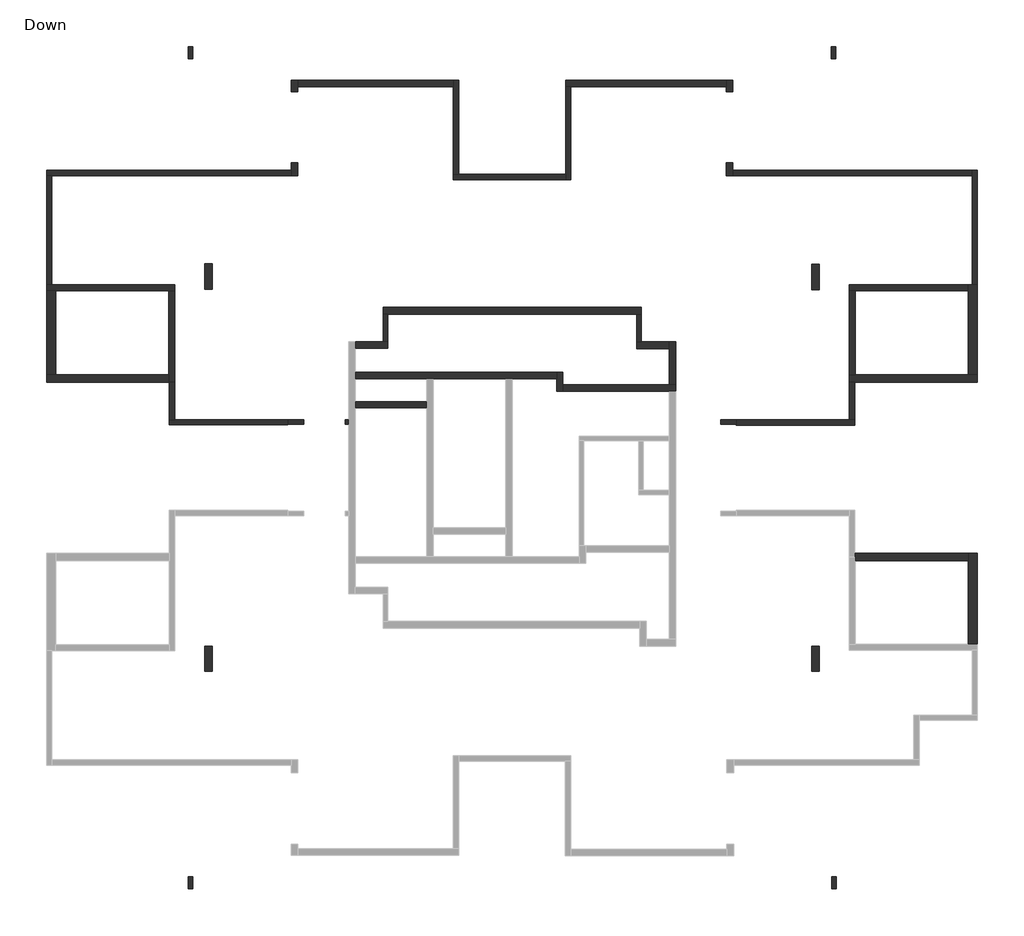
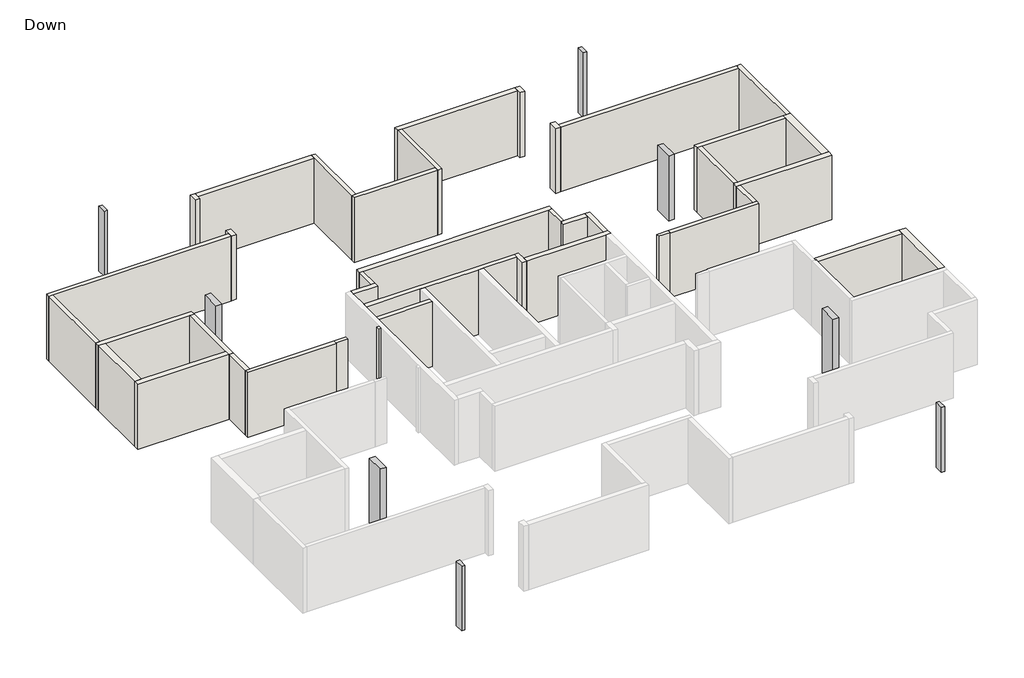
# One storey, part 2 of 2: 40 walls, 8 columns.
# Revit data of these elements (continued)
# Element 36 (IfcWall, "22") (continued)
#   SOFiSTiK_AMG_Comments = ""
#   Top Offset = 0 cm
#   Base Offset = 0 cm
#   wall height = 307 cm
#   SOFiSTiK_AMG_Scheduled = yes
#   SOFiSTiK_AMG_Adjusted = yes
#   Phase Created = New Construction
#   Base Constraint = Down
#   Top Constraint = Typical Floor
#   Materials on its faces: "Concrete"
# Element 37 (IfcWall, "22")
#   Comments = ""
#   Mark = "W51"
#   SOFiSTiK_EdgeZones = "W51"
#   SOFiSTiK_AMG_Comments = ""
#   Top Offset = 0 cm
#   Base Offset = 0 cm
#   wall height = 307 cm
#   SOFiSTiK_AMG_Scheduled = yes
#   SOFiSTiK_AMG_Adjusted = yes
#   Phase Created = New Construction
#   Base Constraint = Down
#   Top Constraint = Typical Floor
#   Materials on its faces: "Concrete"
# Element 38 (IfcWall, "22")
#   Comments = ""
#   Mark = "W52"
#   SOFiSTiK_EdgeZones = "W52"
#   SOFiSTiK_AMG_Comments = ""
#   Top Offset = 0 cm
#   Base Offset = 0 cm
#   wall height = 307 cm
#   SOFiSTiK_AMG_Scheduled = yes
#   SOFiSTiK_AMG_Adjusted = yes
#   Phase Created = New Construction
#   Base Constraint = Down
#   Top Constraint = Typical Floor
#   Materials on its faces: "Concrete"
# Element 39 (IfcWall, "22")
#   Comments = ""
#   Mark = "W64"
#   SOFiSTiK_EdgeZones = "W64"
#   SOFiSTiK_AMG_Comments = ""
#   Top Offset = 0 cm
#   Base Offset = 0 cm
#   wall height = 307 cm
#   SOFiSTiK_AMG_Scheduled = yes
#   SOFiSTiK_AMG_Adjusted = yes
#   Phase Created = New Construction
#   Base Constraint = Down
#   Top Constraint = Typical Floor
#   Materials on its faces: "Concrete"
# Element 40 (IfcWall, "22")
#   Comments = ""
#   Mark = "W65"
#   SOFiSTiK_EdgeZones = "W65"
#   SOFiSTiK_AMG_Comments = ""
#   Top Offset = 0 cm
#   Base Offset = 0 cm
#   wall height = 307 cm
#   SOFiSTiK_AMG_Scheduled = yes
#   SOFiSTiK_AMG_Adjusted = yes
#   Phase Created = New Construction
#   Base Constraint = Down
#   Top Constraint = Typical Floor
#   Materials on its faces: "Concrete"
# Element 41 (IfcWall, "22")
#   Comments = ""
#   Mark = "W66"
#   SOFiSTiK_EdgeZones = "W66"
#   SOFiSTiK_AMG_Comments = ""
#   Top Offset = 0 cm
#   Base Offset = 0 cm
#   wall height = 307 cm
#   SOFiSTiK_AMG_Scheduled = yes
#   SOFiSTiK_AMG_Adjusted = yes
#   Phase Created = New Construction
#   Base Constraint = Down
#   Top Constraint = Typical Floor
#   Materials on its faces: "Concrete"
# Element 42 (IfcWall, "22")
#   Comments = ""
#   Mark = "W67"
#   SOFiSTiK_EdgeZones = "W67"
#   SOFiSTiK_AMG_Comments = ""
#   Top Offset = 0 cm
#   Base Offset = 0 cm
#   wall height = 307 cm
#   SOFiSTiK_AMG_Scheduled = yes
#   SOFiSTiK_AMG_Adjusted = yes
#   Phase Created = New Construction
#   Base Constraint = Down
#   Top Constraint = Typical Floor
#   Materials on its faces: "Concrete"
# Element 43 (IfcWall, "25")
#   Comments = ""
#   Mark = "W30"
#   SOFiSTiK_EdgeZones = "W30"
#   SOFiSTiK_AMG_Comments = ""
#   Top Offset = 0 cm
#   Base Offset = 0 cm
#   wall height = 307 cm
#   SOFiSTiK_AMG_Scheduled = yes
#   SOFiSTiK_AMG_Adjusted = yes
#   Phase Created = New Construction
#   Base Constraint = Down
#   Top Constraint = Typical Floor
#   Materials on its faces: "Concrete"
# Element 44 (IfcWall, "25")
#   Comments = ""
#   Mark = "W31"
#   SOFiSTiK_EdgeZones = "W31"
#   SOFiSTiK_AMG_Comments = ""
#   Top Offset = 0 cm
#   Base Offset = 0 cm
#   wall height = 307 cm
#   SOFiSTiK_AMG_Scheduled = yes
#   SOFiSTiK_AMG_Adjusted = yes
#   Phase Created = New Construction
#   Base Constraint = Down
#   Top Constraint = Typical Floor
#   Materials on its faces: "Concrete"
# Element 45 (IfcWall, "25")
#   Comments = ""
#   Mark = "W32"
#   SOFiSTiK_EdgeZones = "W32"
#   SOFiSTiK_AMG_Comments = ""
#   Top Offset = 0 cm
#   Base Offset = 0 cm
#   wall height = 307 cm
#   SOFiSTiK_AMG_Scheduled = yes
#   SOFiSTiK_AMG_Adjusted = yes
#   Phase Created = New Construction
#   Base Constraint = Down
#   Top Constraint = Typical Floor
#   Materials on its faces: "Concrete"
# Element 46 (IfcWall, "30")
#   Comments = ""
#   Mark = "W2"
#   SOFiSTiK_EdgeZones = "W2"
#   SOFiSTiK_AMG_Comments = ""
#   Top Offset = 0 cm
#   Base Offset = 0 cm
#   wall height = 307 cm
#   SOFiSTiK_AMG_Scheduled = yes
#   SOFiSTiK_AMG_Adjusted = yes
#   Phase Created = New Construction
#   Base Constraint = Down
#   Top Constraint = Typical Floor
#   Materials on its faces: "Concrete"
# Element 47 (IfcWall, "30")
#   Comments = ""
#   Mark = "W3"
#   SOFiSTiK_EdgeZones = "W3"
#   SOFiSTiK_AMG_Comments = ""
#   Top Offset = 0 cm
#   Base Offset = 0 cm
#   wall height = 307 cm
#   SOFiSTiK_AMG_Scheduled = yes
#   SOFiSTiK_AMG_Adjusted = yes
#   Phase Created = New Construction
#   Base Constraint = Down
#   Top Constraint = Typical Floor
#   Materials on its faces: "Concrete"
# Element 48 (IfcWall, "30")
#   Comments = ""
#   Mark = "W4"
#   SOFiSTiK_EdgeZones = "W4"
#   SOFiSTiK_AMG_Comments = ""
#   Top Offset = 0 cm
#   Base Offset = 0 cm
#   wall height = 307 cm
#   SOFiSTiK_AMG_Scheduled = yes
#   SOFiSTiK_AMG_Adjusted = yes
#   Phase Created = New Construction
#   Base Constraint = Down
#   Top Constraint = Typical Floor
#   Materials on its faces: "Concrete"
# Materials
#   "Concrete, Cast-in-Place - B30": class "Concrete", colour RGB 192 192 192, transparency 0, Keynote = "01000", Description = "Cast-in-place concrete", Cost = 0
#   "Concrete": class "Concrete", colour RGB 192 192 192, transparency 0, Keynote = "01000", Description = "Cast-in-place concrete", Cost = 0
